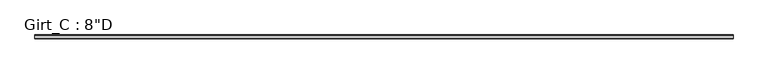
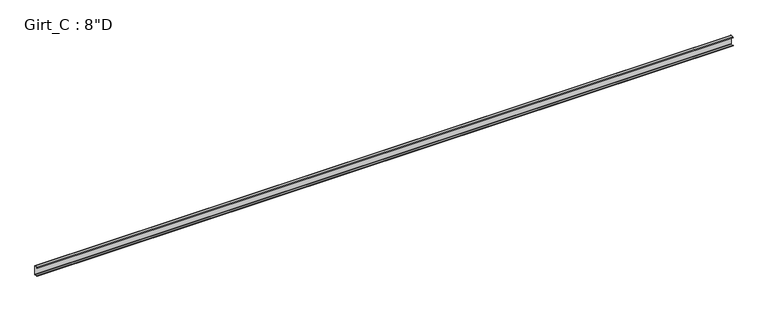
"""IFC4 building model written with IfcOpenShell, lengths in millimetres: beam geometry."""

from ifc_helpers import new_model, si_unit, point, frame, frame_2d, origin, place, context, project, spatial, polyline, circle_curve, trimmed, segment, composite_curve, outline, extrude, source, transform, mapped, element, save


def beam_ff55a9a6(model_context):
    return source(origin(), model_context, "Body", "SweptSolid", [
        extrude(outline(composite_curve([segment(polyline([(-63.5, 101.6), (-3.3734375, 101.6)]), True, "CONTINUOUS"), segment(trimmed(circle_curve(frame_2d((-3.3734375, 96.8375)), 4.7625), [point((-3.3734375, 101.6))], [point((1.3890625, 96.8375))], False, "CARTESIAN"), True, "CONTINUOUS"), segment(polyline([(1.3890625, 96.8375), (1.3890625, -96.8375)]), True, "CONTINUOUS"), segment(trimmed(circle_curve(frame_2d((-3.3734375, -96.8375)), 4.7625), [point((1.3890625, -96.8375))], [point((-3.3734375, -101.6))], False, "CARTESIAN"), True, "CONTINUOUS"), segment(polyline([(-3.3734375, -101.6), (-63.5, -101.6), (-75.745104, -87.0068534), (-73.6169367, -85.221109), (-62.204539, -98.821875), (-3.2694106, -98.821875)]), True, "CONTINUOUS"), segment(trimmed(circle_curve(frame_2d((-3.3748024, -96.8389339)), 1.9857399), [point((-3.2694106, -98.821875))], [point((-1.3890625, -96.8389339))], True, "CARTESIAN"), True, "CONTINUOUS"), segment(polyline([(-1.3890625, -96.8389339), (-1.3890625, 96.8381931)]), True, "CONTINUOUS"), segment(trimmed(circle_curve(frame_2d((-3.3741066, 96.8381931)), 1.9850441), [point((-1.3890625, 96.8381931))], [point((-3.3005807, 98.821875))], True, "CARTESIAN"), True, "CONTINUOUS"), segment(polyline([(-3.3005807, 98.821875), (-62.204539, 98.821875), (-73.6169367, 85.221109), (-75.745104, 87.0068534), (-63.5, 101.6)]), True, "CONTINUOUS")], self_intersect=False)), frame((-7289.7527498, 0.0, 0.0), z_axis=(1.0, 0.0, 0.0), x_axis=(0.0, 1.0, 0.0)), (0.0, 0.0, 1.0), 14538.2144519),
    ])


if __name__ == "__main__":
    model = new_model("IFC4")
    model_context = context("Model", 3, world=origin())
    ifc_project = project(units=[si_unit("LENGTHUNIT", "METRE", prefix="MILLI")], contexts=[model_context])
    site = spatial("IfcSite", under=ifc_project)
    building = spatial("IfcBuilding", under=site)
    placement = place(None, origin())
    beam_shape = beam_ff55a9a6(model_context)
    element("IfcBeam", 1, ObjectType="Girt_C : 8\"D", at=placement, inside=building, context=model_context, shape_type="MappedRepresentation", body=[
        mapped(beam_shape, transform((0.0, 0.0, 0.0), x_axis=(1.0, 0.0, 0.0), y_axis=(0.0, 1.0, 0.0), z_axis=(0.0, 0.0, 1.0))),
    ])
    save(model, "model.ifc")

# Revit data of these elements
# Type "Girt_C : 8\"D"
#   Web_Thickness = 0' - 0 7/64"
#   Length [instance default] = 10' - 0"
#   Leg_1 = 0' - 2 1/2"
#   Height = 0' - 8"
#   Structural Material [instance default] = none
